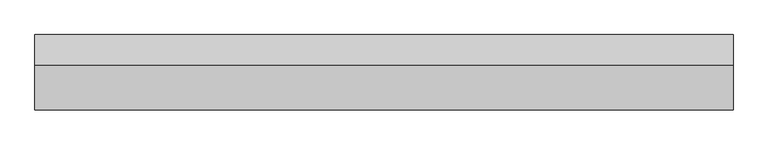
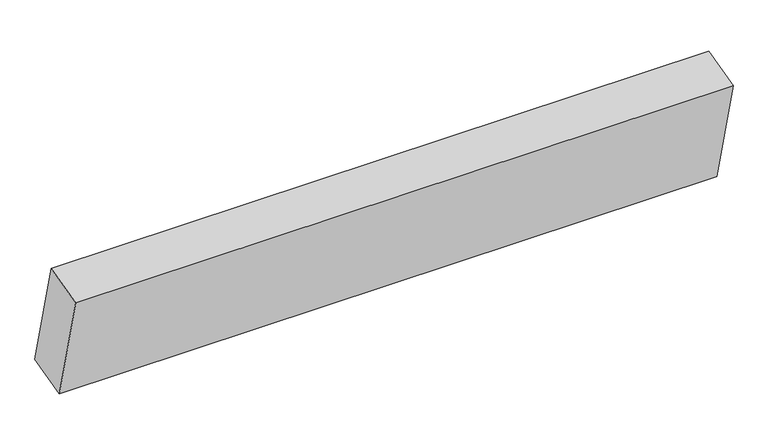
"""IFC4 building model written with IfcOpenShell, lengths in millimetres: proxy geometry, Structure005 575 : Structure005 575."""

from ifc_helpers import new_model, si_unit, frame, origin, place, context, project, spatial, polyline, outline, extrude, source, transform, mapped, element, save


def generic_models_1d49aaba(model_context):
    return source(origin(), model_context, "Body", "SweptSolid", [
        extrude(outline(polyline([(0.0, -133.35), (0.0, 0.0), (2000.0, 0.0), (2000.0, -133.35), (0.0, -133.35)])), frame((3694.2883192, 10746.1792758, 43490.2459395), z_axis=(0.0, -0.24259923079540666, 0.9701265964901061), x_axis=(1.0, 0.0, 0.0)), (0.0, 0.0, 1.0), 355.6),
    ])


if __name__ == "__main__":
    model = new_model("IFC4")
    model_context = context("Model", 3, world=origin())
    ifc_project = project(units=[si_unit("LENGTHUNIT", "METRE", prefix="MILLI")], contexts=[model_context])
    site = spatial("IfcSite", under=ifc_project)
    building = spatial("IfcBuilding", under=site)
    placement = place(None, origin())
    generic_models_shape = generic_models_1d49aaba(model_context)
    element("IfcBuildingElementProxy", 1, Name="Structure005 575 : Structure005 575", ObjectType="Structure005 575 : Structure005 575", at=placement, inside=building, context=model_context, shape_type="MappedRepresentation", body=[
        mapped(generic_models_shape, transform((0.0, 0.0, 0.0), x_axis=(1.0, 0.0, 0.0), y_axis=(0.0, 1.0, 0.0), z_axis=(0.0, 0.0, 1.0))),
    ])
    save(model, "model.ifc")

# Revit data of these elements
# Type "Structure005 575 : Structure005 575"
#   NameOverride = "Structure005"
# Element 1 (IfcBuildingElementProxy, "Structure005 575 : Structure005 575")
#   Materials on its faces: "STRUCTURAL MEMBER (SEE STRUCTURAL DWGS)"
# Materials
#   "STRUCTURAL MEMBER (SEE STRUCTURAL DWGS)": class "Unassigned", colour RGB 176 134 95, transparency 0, Cost = 0
